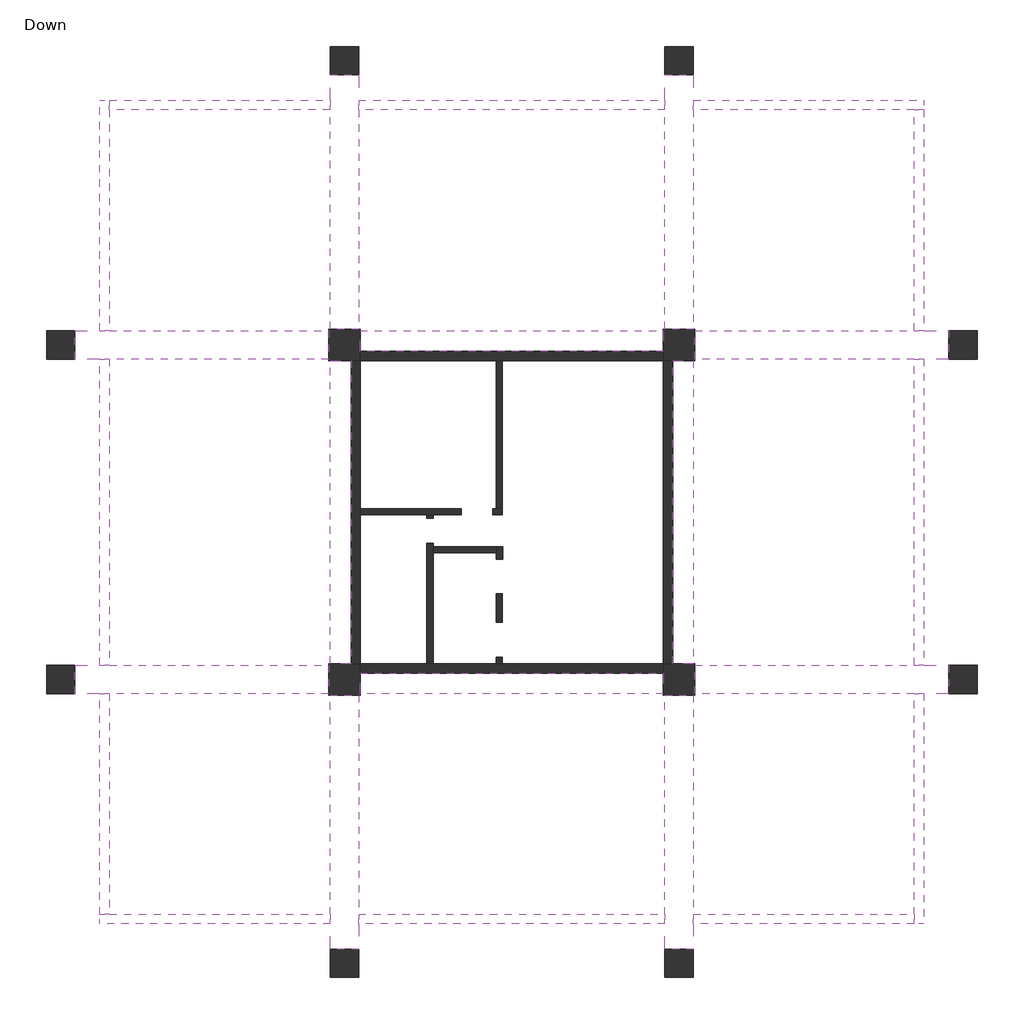
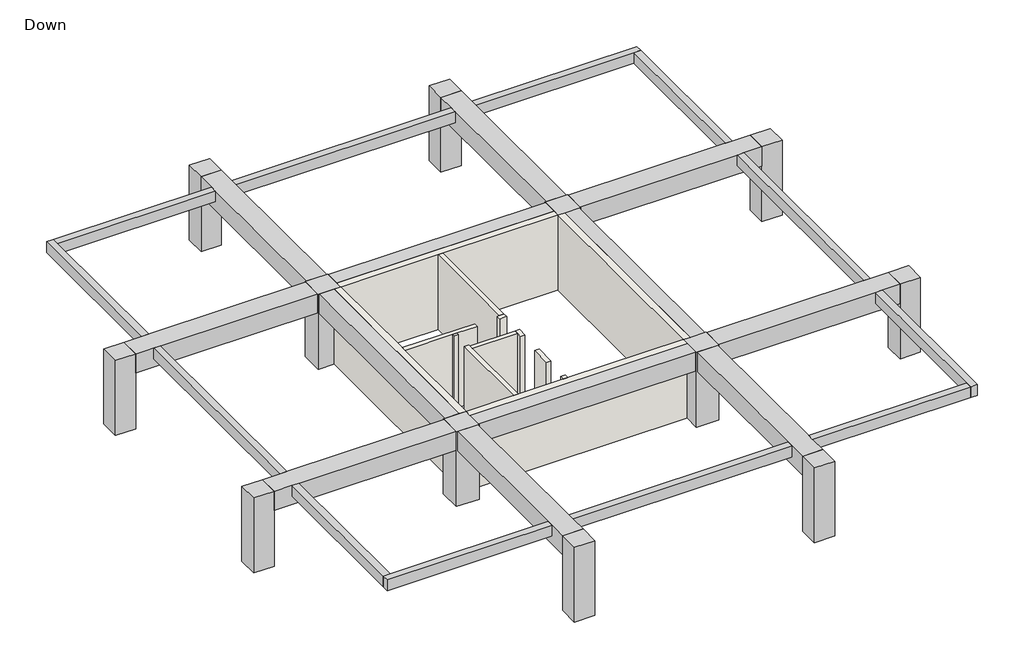
# One storey: 24 beams, 13 walls, 12 columns.
# Revit data of these elements (continued)
# Element 20 (IfcBeam, "Concrete Rectengular Beam : 90/90") (continued)
#   SOFiSTiK_AMG_Comments = ""
#   SOFiSTiK_AMG_Scheduled = yes
#   SOFiSTiK_AMG_Adjusted = yes
#   Structural Material = Concrete
#   Phase Created = New Construction
#   Materials on its faces: "Concrete"
# Element 21 (IfcBeam, "Concrete Rectengular Beam : 90/90")
#   Comments = ""
#   Mark = "B21"
#   SOFiSTiK_AMG_Comments = ""
#   SOFiSTiK_AMG_Scheduled = yes
#   SOFiSTiK_AMG_Adjusted = yes
#   Structural Material = Concrete
#   Phase Created = New Construction
#   Materials on its faces: "Concrete"
# Element 22 (IfcBeam, "Concrete Rectengular Beam : 90/90")
#   Comments = ""
#   Mark = "B22"
#   SOFiSTiK_AMG_Comments = ""
#   SOFiSTiK_AMG_Scheduled = yes
#   SOFiSTiK_AMG_Adjusted = yes
#   Structural Material = Concrete
#   Phase Created = New Construction
#   Materials on its faces: "Concrete"
# Element 23 (IfcBeam, "Concrete Rectengular Beam : 90/90")
#   Comments = ""
#   Mark = "B23"
#   SOFiSTiK_AMG_Comments = ""
#   SOFiSTiK_AMG_Scheduled = yes
#   SOFiSTiK_AMG_Adjusted = yes
#   Structural Material = Concrete
#   Phase Created = New Construction
#   Materials on its faces: "Concrete"
# Element 24 (IfcBeam, "Concrete Rectengular Beam : 90/90")
#   Comments = ""
#   Mark = "B24"
#   SOFiSTiK_AMG_Comments = ""
#   SOFiSTiK_AMG_Scheduled = yes
#   SOFiSTiK_AMG_Adjusted = yes
#   Structural Material = Concrete
#   Phase Created = New Construction
#   Materials on its faces: "Concrete"
# Element 25 (IfcColumn, "Concrete Rectengular Column : 100/100")
#   Comments = ""
#   Mark = "C1"
#   SOFiSTiK_AMG_Comments = ""
#   SOFiSTiK_AMG_Scheduled = yes
#   SOFiSTiK_AMG_Adjusted = yes
#   Structural Material = Concrete
#   Phase Created = New Construction
#   Materials on its faces: "Concrete"
# Element 26 (IfcColumn, "Concrete Rectengular Column : 100/100")
#   Comments = ""
#   Mark = "C2"
#   SOFiSTiK_AMG_Comments = ""
#   SOFiSTiK_AMG_Scheduled = yes
#   SOFiSTiK_AMG_Adjusted = yes
#   Structural Material = Concrete
#   Phase Created = New Construction
#   Materials on its faces: "Concrete"
# Element 27 (IfcColumn, "Concrete Rectengular Column : 100/100")
#   Comments = ""
#   Mark = "C3"
#   SOFiSTiK_AMG_Comments = ""
#   SOFiSTiK_AMG_Scheduled = yes
#   SOFiSTiK_AMG_Adjusted = yes
#   Structural Material = Concrete
#   Phase Created = New Construction
#   Materials on its faces: "Concrete"
# Element 28 (IfcColumn, "Concrete Rectengular Column : 100/100")
#   Comments = ""
#   Mark = "C4"
#   SOFiSTiK_AMG_Comments = ""
#   SOFiSTiK_AMG_Scheduled = yes
#   SOFiSTiK_AMG_Adjusted = yes
#   Structural Material = Concrete
#   Phase Created = New Construction
#   Materials on its faces: "Concrete"
# Element 29 (IfcColumn, "Concrete Rectengular Column : 90/90")
#   Comments = ""
#   Mark = "C5"
#   SOFiSTiK_AMG_Comments = ""
#   SOFiSTiK_AMG_Scheduled = yes
#   SOFiSTiK_AMG_Adjusted = yes
#   Structural Material = Concrete
#   Phase Created = New Construction
#   Materials on its faces: "Concrete"
# Element 30 (IfcColumn, "Concrete Rectengular Column : 90/90")
#   Comments = ""
#   Mark = "C6"
#   SOFiSTiK_AMG_Comments = ""
#   SOFiSTiK_AMG_Scheduled = yes
#   SOFiSTiK_AMG_Adjusted = yes
#   Structural Material = Concrete
#   Phase Created = New Construction
#   Materials on its faces: "Concrete"
# Element 31 (IfcColumn, "Concrete Rectengular Column : 90/90")
#   Comments = ""
#   Mark = "C7"
#   SOFiSTiK_AMG_Comments = ""
#   SOFiSTiK_AMG_Scheduled = yes
#   SOFiSTiK_AMG_Adjusted = yes
#   Structural Material = Concrete
#   Phase Created = New Construction
#   Materials on its faces: "Concrete"
# Element 32 (IfcColumn, "Concrete Rectengular Column : 90/90")
#   Comments = ""
#   Mark = "C8"
#   SOFiSTiK_AMG_Comments = ""
#   SOFiSTiK_AMG_Scheduled = yes
#   SOFiSTiK_AMG_Adjusted = yes
#   Structural Material = Concrete
#   Phase Created = New Construction
#   Materials on its faces: "Concrete"
# Element 33 (IfcColumn, "Concrete Rectengular Column : 90/90")
#   Comments = ""
#   Mark = "C9"
#   SOFiSTiK_AMG_Comments = ""
#   SOFiSTiK_AMG_Scheduled = yes
#   SOFiSTiK_AMG_Adjusted = yes
#   Structural Material = Concrete
#   Phase Created = New Construction
#   Materials on its faces: "Concrete"
# Element 34 (IfcColumn, "Concrete Rectengular Column : 90/90")
#   Comments = ""
#   Mark = "C10"
#   SOFiSTiK_AMG_Comments = ""
#   SOFiSTiK_AMG_Scheduled = yes
#   SOFiSTiK_AMG_Adjusted = yes
#   Structural Material = Concrete
#   Phase Created = New Construction
#   Materials on its faces: "Concrete"
# Element 35 (IfcColumn, "Concrete Rectengular Column : 90/90")
#   Comments = ""
#   Mark = "C11"
#   SOFiSTiK_AMG_Comments = ""
#   SOFiSTiK_AMG_Scheduled = yes
#   SOFiSTiK_AMG_Adjusted = yes
#   Structural Material = Concrete
#   Phase Created = New Construction
#   Materials on its faces: "Concrete"
# Element 36 (IfcColumn, "Concrete Rectengular Column : 90/90")
#   Comments = ""
#   Mark = "C12"
#   SOFiSTiK_AMG_Comments = ""
#   SOFiSTiK_AMG_Scheduled = yes
#   SOFiSTiK_AMG_Adjusted = yes
#   Structural Material = Concrete
#   Phase Created = New Construction
#   Materials on its faces: "Concrete"
# Element 37 (IfcWall, "20")
#   Comments = ""
#   Mark = "W5"
#   SOFiSTiK_EdgeZones = "W5"
#   SOFiSTiK_AMG_Comments = ""
#   Top Offset = 0 cm
#   Base Offset = 0 cm
#   wall height = 350 cm
#   SOFiSTiK_AMG_Scheduled = yes
#   SOFiSTiK_AMG_Adjusted = yes
#   Phase Created = New Construction
#   Base Constraint = Down
#   Top Constraint = Typical Floor
#   Materials on its faces: "Concrete"
# Element 38 (IfcWall, "20")
#   Comments = ""
#   Mark = "W6"
#   SOFiSTiK_EdgeZones = "W6"
#   SOFiSTiK_AMG_Comments = "Too Short /"
#   Top Offset = 0 cm
#   Base Offset = 0 cm
#   wall height = 350 cm
#   SOFiSTiK_AMG_Scheduled = yes
#   SOFiSTiK_AMG_Adjusted = yes
#   Phase Created = New Construction
#   Base Constraint = Down
#   Top Constraint = Typical Floor
#   Materials on its faces: "Concrete"
# Element 39 (IfcWall, "20")
#   Comments = ""
#   Mark = "W7"
#   SOFiSTiK_EdgeZones = "W7"
#   SOFiSTiK_AMG_Comments = ""
#   Top Offset = 0 cm
#   Base Offset = 0 cm
#   wall height = 350 cm
#   SOFiSTiK_AMG_Scheduled = yes
#   SOFiSTiK_AMG_Adjusted = yes
#   Phase Created = New Construction
#   Base Constraint = Down
#   Top Constraint = Typical Floor
#   Materials on its faces: "Concrete"
# Element 40 (IfcWall, "20")
#   Comments = ""
#   Mark = "W8"
#   SOFiSTiK_EdgeZones = "W8"
#   SOFiSTiK_AMG_Comments = ""
#   Top Offset = 0 cm
#   Base Offset = 0 cm
#   wall height = 350 cm
#   SOFiSTiK_AMG_Scheduled = yes
#   SOFiSTiK_AMG_Adjusted = yes
#   Phase Created = New Construction
#   Base Constraint = Down
#   Top Constraint = Typical Floor
#   Materials on its faces: "Concrete"
# Element 41 (IfcWall, "20")
#   Comments = ""
#   Mark = "W9"
#   SOFiSTiK_EdgeZones = "W9"
#   SOFiSTiK_AMG_Comments = ""
#   Top Offset = 0 cm
#   Base Offset = 0 cm
#   wall height = 350 cm
#   SOFiSTiK_AMG_Scheduled = yes
#   SOFiSTiK_AMG_Adjusted = yes
#   Phase Created = New Construction
#   Base Constraint = Down
#   Top Constraint = Typical Floor
#   Materials on its faces: "Concrete"
# Element 42 (IfcWall, "20")
#   Comments = ""
#   Mark = "W10"
#   SOFiSTiK_EdgeZones = "W10"
#   SOFiSTiK_AMG_Comments = ""
#   Top Offset = 0 cm
#   Base Offset = 0 cm
#   wall height = 350 cm
#   SOFiSTiK_AMG_Scheduled = yes
#   SOFiSTiK_AMG_Adjusted = yes
#   Phase Created = New Construction
#   Base Constraint = Down
#   Top Constraint = Typical Floor
#   Materials on its faces: "Concrete"
# Element 43 (IfcWall, "20")
#   Comments = ""
#   Mark = "W11"
#   SOFiSTiK_EdgeZones = "W11"
#   SOFiSTiK_AMG_Comments = ""
#   Top Offset = 0 cm
#   Base Offset = 0 cm
#   wall height = 350 cm
#   SOFiSTiK_AMG_Scheduled = yes
#   SOFiSTiK_AMG_Adjusted = yes
#   Phase Created = New Construction
#   Base Constraint = Down
#   Top Constraint = Typical Floor
#   Materials on its faces: "Concrete"
# Element 44 (IfcWall, "20")
#   Comments = ""
#   Mark = "W12"
#   SOFiSTiK_EdgeZones = "W12"
#   SOFiSTiK_AMG_Comments = ""
#   Top Offset = 0 cm
#   Base Offset = 0 cm
#   wall height = 350 cm
#   SOFiSTiK_AMG_Scheduled = yes
#   SOFiSTiK_AMG_Adjusted = yes
#   Phase Created = New Construction
#   Base Constraint = Down
#   Top Constraint = Typical Floor
#   Materials on its faces: "Concrete"
# Element 45 (IfcWall, "20")
#   Comments = ""
#   Mark = "W13"
#   SOFiSTiK_EdgeZones = "W13"
#   SOFiSTiK_AMG_Comments = ""
#   Top Offset = 0 cm
#   Base Offset = 0 cm
#   wall height = 350 cm
#   SOFiSTiK_AMG_Scheduled = yes
#   SOFiSTiK_AMG_Adjusted = yes
#   Phase Created = New Construction
#   Base Constraint = Down
#   Top Constraint = Typical Floor
#   Materials on its faces: "Concrete"
# Element 46 (IfcWall, "30")
#   Comments = ""
#   Mark = "W1"
#   SOFiSTiK_EdgeZones = "W1"
#   SOFiSTiK_AMG_Comments = ""
#   Top Offset = 0 cm
#   Base Offset = 0 cm
#   wall height = 350 cm
#   SOFiSTiK_AMG_Scheduled = yes
#   SOFiSTiK_AMG_Adjusted = yes
#   Phase Created = New Construction
#   Base Constraint = Down
#   Top Constraint = Typical Floor
#   Materials on its faces: "Concrete"
# Element 47 (IfcWall, "30")
#   Comments = ""
#   Mark = "W2"
#   SOFiSTiK_EdgeZones = "W2"
#   SOFiSTiK_AMG_Comments = ""
#   Top Offset = 0 cm
#   Base Offset = 0 cm
#   wall height = 350 cm
#   SOFiSTiK_AMG_Scheduled = yes
#   SOFiSTiK_AMG_Adjusted = yes
#   Phase Created = New Construction
#   Base Constraint = Down
#   Top Constraint = Typical Floor
#   Materials on its faces: "Concrete"
# Element 48 (IfcWall, "30")
#   Comments = ""
#   Mark = "W3"
#   SOFiSTiK_EdgeZones = "W3"
#   SOFiSTiK_AMG_Comments = ""
#   Top Offset = 0 cm
#   Base Offset = 0 cm
#   wall height = 350 cm
#   SOFiSTiK_AMG_Scheduled = yes
#   SOFiSTiK_AMG_Adjusted = yes
#   Phase Created = New Construction
#   Base Constraint = Down
#   Top Constraint = Typical Floor
#   Materials on its faces: "Concrete"
# Element 49 (IfcWall, "30")
#   Comments = ""
#   Mark = "W4"
#   SOFiSTiK_EdgeZones = "W4"
#   SOFiSTiK_AMG_Comments = ""
#   Top Offset = 0 cm
#   Base Offset = 0 cm
#   wall height = 350 cm
#   SOFiSTiK_AMG_Scheduled = yes
#   SOFiSTiK_AMG_Adjusted = yes
#   Phase Created = New Construction
#   Base Constraint = Down
#   Top Constraint = Typical Floor
#   Materials on its faces: "Concrete"
# Materials
#   "Concrete": class "Concrete", colour RGB 192 192 192, transparency 0, Keynote = "01000", Description = "Cast-in-place concrete", Cost = 0
